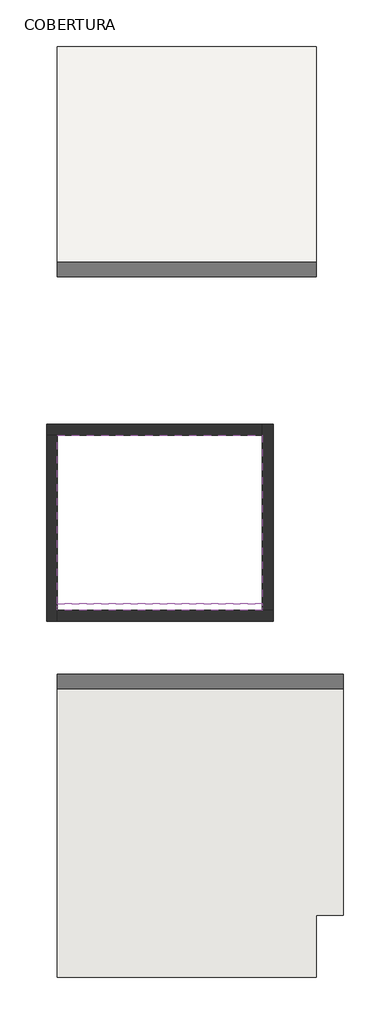
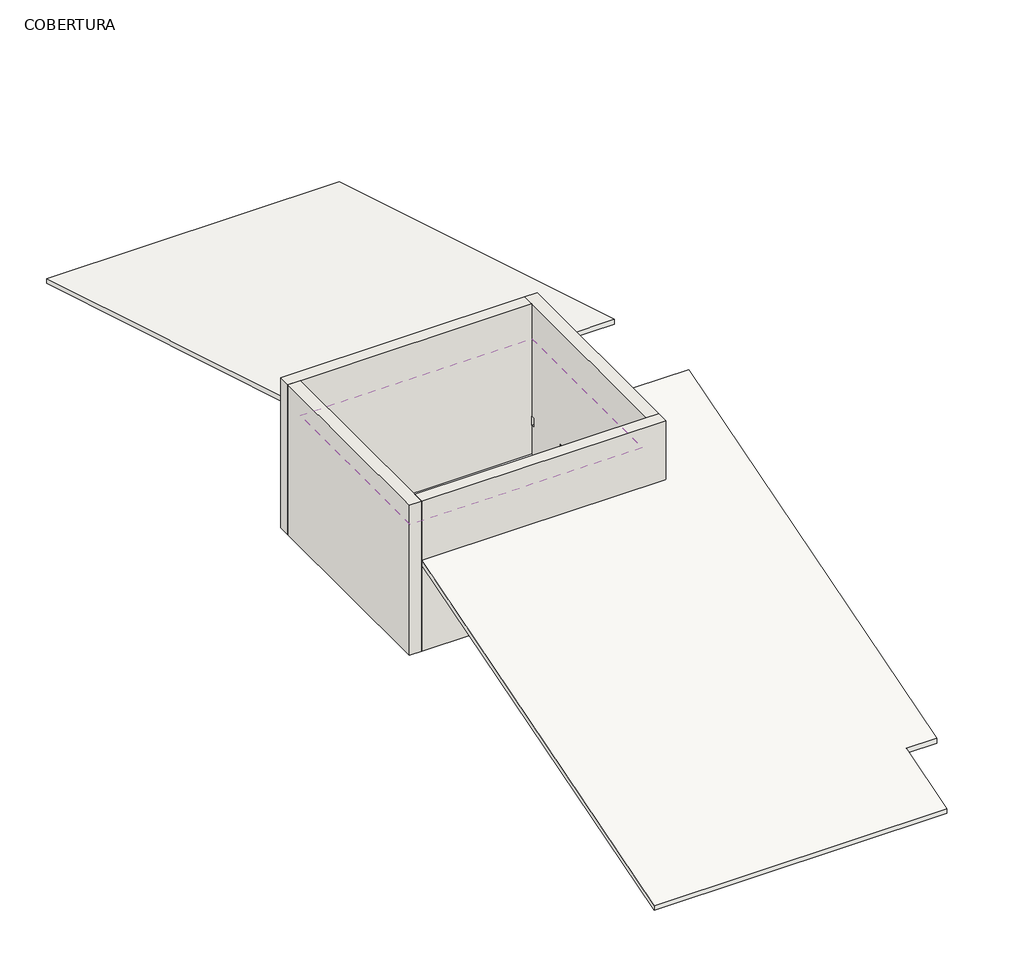
# One storey: 4 walls, 3 roofs, 1 pipe segment.
"""IFC4 building model written with IfcOpenShell, lengths in millimetres."""

from ifc_helpers import new_model, si_unit, frame, origin, place, context, project, spatial, polyline, outline, extrude, faceted_brep, element, save

model = new_model("IFC4")

# Units and contexts
model_context = context("Model", 3, world=origin())
ifc_project = project(units=[si_unit("LENGTHUNIT", "METRE", prefix="MILLI")], contexts=[model_context])

# Site, building, storey
site = spatial("IfcSite", under=ifc_project)
building = spatial("IfcBuilding", under=site)
storey = spatial("IfcBuildingStorey", under=building, Name="COBERTURA", Elevation=6160.0)

# Pipe segment
placement = place(None, origin())
element("IfcPipeSegment", 1, ObjectType=".CALHA 12.5 cm", at=placement, inside=storey, context=model_context, shape_type="SweptSolid", body=[
    extrude(outline(polyline([(-2115.2624019, 8115.4867724), (-2189.4624019, 8115.4867724), (-2227.5624019, 8214.999005), (-2240.2624019, 8214.999005), (-2240.2624019, 8227.699005), (-2227.5624019, 8227.699005), (-2227.5624019, 8224.524005), (-2237.0874019, 8224.524005), (-2237.0874019, 8218.174005), (-2225.2001046, 8218.174005), (-2187.1001046, 8118.6617724), (-2118.4374019, 8118.6617724), (-2118.4374019, 8240.399005), (-2115.2624019, 8240.399005), (-2115.2624019, 8115.4867724)])), frame((-2574.4431325, 0.0, 0.0), z_axis=(1.0, 0.0, 0.0), x_axis=(0.0, 1.0, 0.0)), (0.0, 0.0, 1.0), 3800.0),
])

# Roofs
element("IfcRoof", 2, ObjectType="TELHA METÁLICA", at=placement, inside=storey, context=model_context, shape_type="SweptSolid", body=[
    extrude(outline(polyline([(-2115.2624019, 8240.399005), (1009.7375981, 8552.899005), (1009.7375981, 8472.5), (-2115.2624019, 8160.0), (-2115.2624019, 8240.399005)])), frame((-2574.4431325, 0.0, 0.0), z_axis=(1.0, 0.0, 0.0), x_axis=(0.0, 1.0, 0.0)), (0.0, 0.0, 1.0), 3800.0),
])
element("IfcRoof", 3, ObjectType=".TELHA CERÂMICA", at=placement, inside=storey, context=model_context, shape_type="Brep", body=[
    faceted_brep([(-2574.4431325, -2440.2624019, 7655.0), (1425.5568675, -2440.2624019, 7655.0), (1425.5568675, -840.2624019, 8135.0), (2725.5568675, -840.2624019, 8135.0), (2725.5568675, -7890.2624019, 6020.0), (2225.5568675, -7890.2624019, 6020.0), (2225.5568675, -9040.2624019, 5675.0), (-2574.4431325, -9040.2624019, 5675.0), (1425.5568675, -2440.2624019, 7738.5224521), (-2574.4431325, -2440.2624019, 7738.5224521), (-2574.4431325, -9040.2624019, 5758.5224521), (2225.5568675, -9040.2624019, 5758.5224521), (2225.5568675, -7890.2624019, 6103.5224521), (2725.5568675, -7890.2624019, 6103.5224521), (2725.5568675, -840.2624019, 8218.5224521), (1425.5568675, -840.2624019, 8218.5224521)], [[[0, 1, 2, 3, 4, 5, 6, 7]], [[8, 9, 10, 11, 12, 13, 14, 15]], [[6, 11, 10, 7]], [[9, 8, 1, 0]], [[10, 9, 0, 7]], [[14, 13, 4, 3]], [[15, 14, 3, 2]], [[8, 15, 2, 1]], [[12, 11, 6, 5]], [[13, 12, 5, 4]]]),
])
element("IfcRoof", 4, ObjectType=".TELHA CERÂMICA", at=placement, inside=storey, context=model_context, shape_type="Brep", body=[
    faceted_brep([(1425.5568675, 1209.7375981, 8180.0), (-2574.4431325, 1209.7375981, 8180.0), (-2574.4431325, 8209.7375981, 6080.0), (2225.5568675, 8209.7375981, 6080.0), (2225.5568675, 409.7375981, 8420.0), (1425.5568675, 409.7375981, 8420.0), (-2574.4431325, 1209.7375981, 8263.5224521), (1425.5568675, 1209.7375981, 8263.5224521), (1425.5568675, 409.7375981, 8503.5224521), (2225.5568675, 409.7375981, 8503.5224521), (2225.5568675, 8209.7375981, 6163.5224521), (-2574.4431325, 8209.7375981, 6163.5224521)], [[[0, 1, 2, 3, 4, 5]], [[6, 7, 8, 9, 10, 11]], [[2, 11, 10, 3]], [[7, 6, 1, 0]], [[6, 11, 2, 1]], [[10, 9, 4, 3]], [[8, 7, 0, 5]], [[9, 8, 5, 4]]]),
])

# Walls
element("IfcWall", 5, ObjectType=".EXT. PAREDE 20 cm - PINTURA/PINTURA", at=placement, inside=storey, context=model_context, shape_type="Brep", body=[
    faceted_brep([(-2774.4431325, 1009.7375981, 8760.0), (-2774.4431325, 1009.7375981, 6160.0), (-2574.4431325, 1009.7375981, 6160.0), (1225.5568675, 1009.7375981, 6160.0), (1225.5568675, 1009.7375981, 6660.0), (1225.5568675, 1009.7375981, 6810.0), (1225.5568675, 1009.7375981, 6830.0), (1225.5568675, 1009.7375981, 8760.0), (-2574.4431325, 1009.7375981, 8760.0), (-2774.4431325, 1209.7375981, 6160.0), (-2774.4431325, 1209.7375981, 7542.5413482), (-2774.4431325, 1209.7375981, 8472.3285822), (-2774.4431325, 1209.7375981, 8760.0), (1225.5568675, 1209.7375981, 8760.0), (1225.5568675, 1209.7375981, 6160.0), (-2574.4431325, 1209.7375981, 6160.0)], [[[0, 1, 2, 3, 4, 5, 6, 7, 8]], [[9, 10, 11, 12, 13, 14, 15]], [[3, 2, 1, 9, 15, 14]], [[0, 8, 7, 13, 12]], [[3, 14, 13, 7, 6, 5, 4]], [[0, 12, 11, 10, 9, 1]]]),
])
element("IfcWall", 6, ObjectType=".EXT. PAREDE 20 cm - PINTURA/PINTURA", at=placement, inside=storey, context=model_context, shape_type="Brep", body=[
    faceted_brep([(-2574.4431325, -2440.2624019, 6160.0), (-2574.4431325, -2240.2624019, 6160.0), (-2574.4431325, 1009.7375981, 6160.0), (-2574.4431325, 1009.7375981, 6660.0), (-2574.4431325, 959.7375981, 6660.0), (-2574.4431325, 959.7375981, 6810.0), (-2574.4431325, 1009.7375981, 6810.0), (-2574.4431325, 1009.7375981, 6830.0), (-2574.4431325, 1009.7375981, 8760.0), (-2574.4431325, -2240.2624019, 8760.0), (-2574.4431325, -2440.2624019, 8760.0), (-2574.4431325, -2440.2624019, 7947.3285822), (-2574.4431325, -1440.2624019, 6810.0), (-2574.4431325, -1390.2624019, 6810.0), (-2574.4431325, -1390.2624019, 6660.0), (-2574.4431325, -1440.2624019, 6660.0), (-2574.4431325, -640.2624019, 6810.0), (-2574.4431325, -590.2624019, 6810.0), (-2574.4431325, -590.2624019, 6660.0), (-2574.4431325, -640.2624019, 6660.0), (-2574.4431325, 159.7375981, 6810.0), (-2574.4431325, 209.7375981, 6810.0), (-2574.4431325, 209.7375981, 6660.0), (-2574.4431325, 159.7375981, 6660.0), (-2574.4431325, -2240.2624019, 6810.0), (-2574.4431325, -2190.2624019, 6810.0), (-2574.4431325, -2190.2624019, 6660.0), (-2574.4431325, -2240.2624019, 6660.0), (-2774.4431325, 1009.7375981, 6160.0), (-2774.4431325, -2440.2624019, 6160.0), (-2774.4431325, -2440.2624019, 7947.3285822), (-2774.4431325, -2440.2624019, 8760.0), (-2774.4431325, 1009.7375981, 8760.0), (-2749.4431325, -2440.2624019, 6160.0), (-2724.4431325, -1440.2624019, 6810.0), (-2724.4431325, -1390.2624019, 6810.0), (-2724.4431325, -1390.2624019, 6660.0), (-2724.4431325, -1440.2624019, 6660.0), (-2724.4431325, -640.2624019, 6810.0), (-2724.4431325, -590.2624019, 6810.0), (-2724.4431325, -590.2624019, 6660.0), (-2724.4431325, -640.2624019, 6660.0), (-2724.4431325, 159.7375981, 6810.0), (-2724.4431325, 209.7375981, 6810.0), (-2724.4431325, 209.7375981, 6660.0), (-2724.4431325, 159.7375981, 6660.0), (-2724.4431325, -2240.2624019, 6810.0), (-2724.4431325, -2190.2624019, 6810.0), (-2724.4431325, -2190.2624019, 6660.0), (-2724.4431325, -2240.2624019, 6660.0), (-2724.4431325, 959.7375981, 6810.0), (-2724.4431325, 1009.7375981, 6810.0), (-2724.4431325, 1009.7375981, 6660.0), (-2724.4431325, 959.7375981, 6660.0)], [[[0, 1, 2, 3, 4, 5, 6, 7, 8, 9, 10, 11], [12, 13, 14, 15], [16, 17, 18, 19], [20, 21, 22, 23], [24, 25, 26, 27]], [[28, 29, 30, 31, 32]], [[2, 1, 0, 33, 29, 28]], [[10, 9, 8, 32, 31]], [[10, 31, 30, 29, 33, 0, 11]], [[34, 35, 13, 12]], [[36, 37, 15, 14]], [[35, 36, 14, 13]], [[35, 34, 37, 36]], [[37, 34, 12, 15]], [[38, 39, 17, 16]], [[40, 41, 19, 18]], [[39, 40, 18, 17]], [[39, 38, 41, 40]], [[41, 38, 16, 19]], [[42, 43, 21, 20]], [[44, 45, 23, 22]], [[43, 44, 22, 21]], [[43, 42, 45, 44]], [[45, 42, 20, 23]], [[46, 47, 25, 24]], [[48, 49, 27, 26]], [[47, 48, 26, 25]], [[47, 46, 49, 48]], [[49, 46, 24, 27]], [[50, 51, 6, 5]], [[52, 53, 4, 3]], [[51, 50, 53, 52]], [[53, 50, 5, 4]], [[2, 28, 32, 8, 7, 6, 51, 52, 3]]]),
])
element("IfcWall", 7, ObjectType=".EXT. PAREDE 20 cm - PINTURA/PINTURA", at=placement, inside=storey, context=model_context, shape_type="Brep", body=[
    faceted_brep([(1425.5568675, -2240.2624019, 6160.0), (1225.5568675, -2240.2624019, 6160.0), (-2574.4431325, -2240.2624019, 6160.0), (-2574.4431325, -2240.2624019, 6660.0), (-2574.4431325, -2240.2624019, 6810.0), (-2574.4431325, -2240.2624019, 6830.0), (-2574.4431325, -2240.2624019, 8760.0), (1225.5568675, -2240.2624019, 8760.0), (1425.5568675, -2240.2624019, 8760.0), (1425.5568675, -2440.2624019, 6160.0), (1425.5568675, -2440.2624019, 8760.0), (-2574.4431325, -2440.2624019, 8760.0), (-2574.4431325, -2440.2624019, 6160.0)], [[[0, 1, 2, 3, 4, 5, 6, 7, 8]], [[9, 10, 11, 12]], [[2, 1, 0, 9, 12]], [[8, 7, 6, 11, 10]], [[0, 8, 10, 9]], [[2, 12, 11, 6, 5, 4, 3]]]),
])
element("IfcWall", 8, ObjectType=".EXT. PAREDE 20 cm - PINTURA/PINTURA", at=placement, inside=storey, context=model_context, shape_type="Brep", body=[
    faceted_brep([(1225.5568675, 1209.7375981, 6160.0), (1225.5568675, 1134.7375981, 6160.0), (1225.5568675, 1009.7375981, 6160.0), (1225.5568675, -240.6624019, 6160.0), (1225.5568675, -2240.2624019, 6160.0), (1225.5568675, -2240.2624019, 6660.0), (1225.5568675, -2190.2624019, 6660.0), (1225.5568675, -2190.2624019, 6810.0), (1225.5568675, -2240.2624019, 6810.0), (1225.5568675, -2240.2624019, 6830.0), (1225.5568675, -2240.2624019, 8760.0), (1225.5568675, 1009.7375981, 8760.0), (1225.5568675, 1209.7375981, 8760.0), (1225.5568675, 1209.7375981, 8180.0), (1225.5568675, 1209.7375981, 7280.0), (1225.5568675, -1390.2624019, 6810.0), (1225.5568675, -1440.2624019, 6810.0), (1225.5568675, -1440.2624019, 6660.0), (1225.5568675, -1390.2624019, 6660.0), (1225.5568675, -590.2624019, 6810.0), (1225.5568675, -640.2624019, 6810.0), (1225.5568675, -640.2624019, 6660.0), (1225.5568675, -590.2624019, 6660.0), (1225.5568675, 209.7375981, 6810.0), (1225.5568675, 159.7375981, 6810.0), (1225.5568675, 159.7375981, 6660.0), (1225.5568675, 209.7375981, 6660.0), (1225.5568675, 1009.7375981, 6810.0), (1225.5568675, 959.7375981, 6810.0), (1225.5568675, 959.7375981, 6660.0), (1225.5568675, 1009.7375981, 6660.0), (1425.5568675, -2240.2624019, 6160.0), (1425.5568675, -240.6624019, 6160.0), (1425.5568675, 1134.7375981, 6160.0), (1425.5568675, 1209.7375981, 6160.0), (1425.5568675, 1209.7375981, 7280.0), (1425.5568675, 1209.7375981, 8180.0), (1425.5568675, 1209.7375981, 8760.0), (1425.5568675, -2240.2624019, 8760.0), (1400.5568675, 1209.7375981, 6160.0), (1375.5568675, -2240.2624019, 6810.0), (1375.5568675, -2240.2624019, 6660.0), (1375.5568675, -1390.2624019, 6810.0), (1375.5568675, -1440.2624019, 6810.0), (1375.5568675, -1440.2624019, 6660.0), (1375.5568675, -1390.2624019, 6660.0), (1375.5568675, -590.2624019, 6810.0), (1375.5568675, -640.2624019, 6810.0), (1375.5568675, -640.2624019, 6660.0), (1375.5568675, -590.2624019, 6660.0), (1375.5568675, 209.7375981, 6810.0), (1375.5568675, 159.7375981, 6810.0), (1375.5568675, 159.7375981, 6660.0), (1375.5568675, 209.7375981, 6660.0), (1375.5568675, -2190.2624019, 6810.0), (1375.5568675, -2190.2624019, 6660.0), (1375.5568675, 1009.7375981, 6810.0), (1375.5568675, 959.7375981, 6810.0), (1375.5568675, 959.7375981, 6660.0), (1375.5568675, 1009.7375981, 6660.0)], [[[0, 1, 2, 3, 4, 5, 6, 7, 8, 9, 10, 11, 12, 13, 14], [15, 16, 17, 18], [19, 20, 21, 22], [23, 24, 25, 26], [27, 28, 29, 30]], [[31, 32, 33, 34, 35, 36, 37, 38]], [[4, 3, 2, 1, 0, 39, 34, 33, 32, 31]], [[12, 11, 10, 38, 37]], [[4, 31, 38, 10, 9, 8, 40, 41, 5]], [[42, 43, 16, 15]], [[44, 45, 18, 17]], [[43, 42, 45, 44]], [[45, 42, 15, 18]], [[43, 44, 17, 16]], [[46, 47, 20, 19]], [[48, 49, 22, 21]], [[47, 46, 49, 48]], [[49, 46, 19, 22]], [[47, 48, 21, 20]], [[50, 51, 24, 23]], [[52, 53, 26, 25]], [[51, 50, 53, 52]], [[53, 50, 23, 26]], [[51, 52, 25, 24]], [[54, 40, 8, 7]], [[41, 55, 6, 5]], [[40, 54, 55, 41]], [[55, 54, 7, 6]], [[56, 57, 28, 27]], [[58, 59, 30, 29]], [[57, 56, 59, 58]], [[59, 56, 27, 30]], [[57, 58, 29, 28]], [[12, 37, 36, 35, 34, 39, 0, 14, 13]]]),
])

save(model, "model.ifc")

# Revit data of these elements
# Project information
#   Desenvolvido por = "Isabela Ribeiro"
#   Empresa = "Cursos Construir"
#   Site = "https://construir.arq.br/"
#   Building Name = "Reforma residencial unifamiliar"
#   Author = "Renato Godoi da Cruz"
#   Área do terreno = "142.50 m²"
#   Taxa de ocupação máxima (TO) = "70.00%"
#   Taxa de permeabilidade mínima (TP) = "10.00%"
#   Coeficiente de aproveitamento máximo (CA) = "4"
#   Coeficiente de aproveitamento mínimo (CA) = "0.15"
#   Coeficiente de aproveitamento básico (CA) = "2"
#   Project Issue Date = "Data de emissão"
#   Project Status = "Status do projeto"
#   Client Name = "RENATO GODOI DA CRUZ"
#   Project Address = "RUA MACHADO DE ASSIS"
#   Project Name = "REFORMA E AMPLIAÇÃO DE UMA RESIDÊNCIA UNIFAMILIAR"
#   Project Number = "0001"
# Type "TELHA METÁLICA"
#   Layers, outside or top first: 0.08 m ".TELHA METÁLICA" (function 1)
# Type ".TELHA CERÂMICA"
#   Layers, outside or top first: 0.08 m ".TELHAS" (function 1)
# Type ".EXT. PAREDE 20 cm - PINTURA/PINTURA"
#   Layers, outside or top first: 0.025 m ".ARGAMASSA + PINTURA BRANCA" (function 5); 0.15 m ".ALVENARIA" (function 1); 0.025 m ".ARGAMASSA + PINTURA BRANCA" (function 5)
# Element 1 (IfcPipeSegment, ".CALHA 12.5 cm")
#   Phase Created = Construção existente
#   Materials on its faces: ".ALUMÍNIO"
# Element 2 (IfcRoof, "TELHA METÁLICA")
#   built-in parameter 1001705 = 28.0607 (stored number, unit not read)
#   built-in parameter 1001710 = 33615
#   Phase Created = Construção existente
#   Materials on its faces: ".TELHA METÁLICA"
# Element 3 (IfcRoof, ".TELHA CERÂMICA")
#   built-in parameter 1001705 = 26.9637 (stored number, unit not read)
#   built-in parameter 1001701 = -1.59121 (stored number, unit not read)
#   built-in parameter 1001710 = 33615
#   Phase Created = Construção existente
#   Materials on its faces: ".TELHAS"
# Element 4 (IfcRoof, ".TELHA CERÂMICA")
#   built-in parameter 1001705 = 27.8987 (stored number, unit not read)
#   built-in parameter 1001701 = -0.262467 (stored number, unit not read)
#   built-in parameter 1001710 = 33615
#   Phase Created = Construção nova
#   Materials on its faces: ".TELHAS"
# Elements 5, 6, 7, 8 (IfcWall, ".EXT. PAREDE 20 cm - PINTURA/PINTURA")
#   Top Offset = 2.88 m
#   Base Offset = 0.00 m
#   Unconnected Height = 2.60 m
#   wall height = 2.60 m
#   Phase Created = Construção existente
#   Base Constraint = COBERTURA
#   Materials on its faces: ".ARGAMASSA + PINTURA BRANCA"
# Materials
#   ".TELHA METÁLICA": class "Genérico", colour RGB 120 120 120, transparency 0, Cost = 0
#   ".TELHAS": class "Genérico", colour RGB 0 0 0, transparency 0, Cost = 0
#   ".ARGAMASSA + PINTURA BRANCA": class "Genérico", colour RGB 255 255 255, transparency 0, Cost = 0
#   ".ALVENARIA": class "Alvenaria", colour RGB 192 192 192, transparency 0, Comments = "m²", Description = "Alvenaria em tijolo comum, bloco cerâmico ou bloco de concreto", Cost = 0
#   ".ALUMÍNIO": class "CC_METAIS", colour RGB 244 244 244, transparency 0, Description = "Material alumínio", Cost = 0
